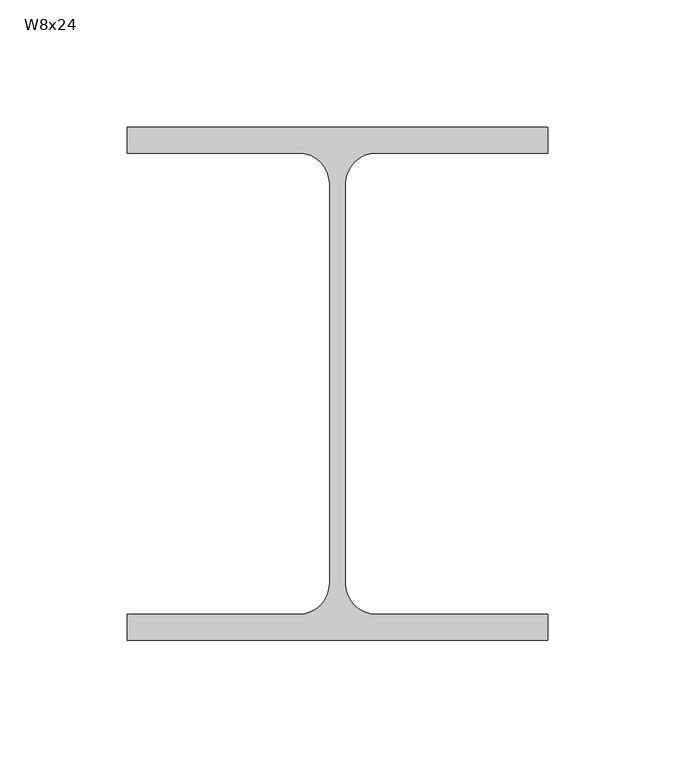
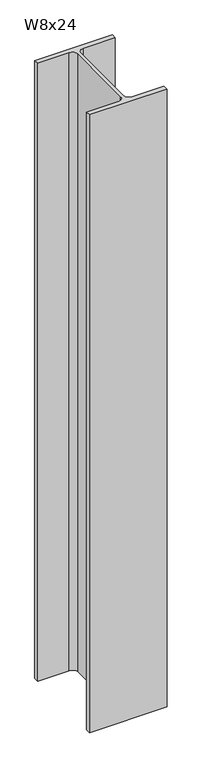
"""IFC4 building model written with IfcOpenShell, lengths in millimetres: column geometry, RME WF - Column : W8x24."""

from ifc_helpers import new_model, si_unit, point, frame, frame_2d, origin, place, context, project, spatial, polyline, circle_curve, trimmed, segment, composite_curve, outline, extrude, source, transform, mapped, element, save


def w8x24_9cd44bdc(model_context):
    return source(origin(), model_context, "Body", "SweptSolid", [
        extrude(outline(composite_curve([segment(polyline([(82.55, 100.711), (82.55, 90.551), (15.1765, 90.551)]), True, "CONTINUOUS"), segment(trimmed(circle_curve(frame_2d((15.1765, 78.486)), 12.065), [point((15.1765, 90.551))], [point((3.1115, 78.486))], True, "CARTESIAN"), True, "CONTINUOUS"), segment(polyline([(3.1115, 78.486), (3.1115, -78.486)]), True, "CONTINUOUS"), segment(trimmed(circle_curve(frame_2d((15.1765, -78.486)), 12.065), [point((3.1115, -78.486))], [point((15.1765, -90.551))], True, "CARTESIAN"), True, "CONTINUOUS"), segment(polyline([(15.1765, -90.551), (82.55, -90.551), (82.55, -100.711), (-82.55, -100.711), (-82.55, -90.551), (-15.1765, -90.551)]), True, "CONTINUOUS"), segment(trimmed(circle_curve(frame_2d((-15.1765, -78.486)), 12.065), [point((-15.1765, -90.551))], [point((-3.1115, -78.486))], True, "CARTESIAN"), True, "CONTINUOUS"), segment(polyline([(-3.1115, -78.486), (-3.1115, 78.486)]), True, "CONTINUOUS"), segment(trimmed(circle_curve(frame_2d((-15.1765, 78.486)), 12.065), [point((-3.1115, 78.486))], [point((-15.1765, 90.551))], True, "CARTESIAN"), True, "CONTINUOUS"), segment(polyline([(-15.1765, 90.551), (-82.55, 90.551), (-82.55, 100.711), (82.55, 100.711)]), True, "CONTINUOUS")], self_intersect=False)), frame((0.0, 0.0, 4699.0), z_axis=(0.0, 0.0, 1.0), x_axis=(1.0, 0.0, 0.0)), (0.0, 0.0, 1.0), 1390.65),
    ])


if __name__ == "__main__":
    model = new_model("IFC4")
    model_context = context("Model", 3, world=origin())
    ifc_project = project(units=[si_unit("LENGTHUNIT", "METRE", prefix="MILLI")], contexts=[model_context])
    site = spatial("IfcSite", under=ifc_project)
    building = spatial("IfcBuilding", under=site)
    placement = place(None, origin())
    w8x24_shape = w8x24_9cd44bdc(model_context)
    element("IfcColumn", 1, ObjectType="RME WF - Column : W8x24", at=placement, inside=building, context=model_context, shape_type="MappedRepresentation", body=[
        mapped(w8x24_shape, transform((0.0, 0.0, 0.0), x_axis=(1.0, 0.0, 0.0), y_axis=(0.0, 1.0, 0.0), z_axis=(0.0, 0.0, 1.0))),
    ])
    save(model, "model.ifc")

# Revit data of these elements
# Type "RME WF - Column : W8x24"
#   Type Mark = "C1"
#   REINF TYPE [instance default] = ""
#   Nominal Size = "W16"
#   COL REMARKS [instance default] = ""
#   BP [instance default] = ""
#   Assembly Code = "B10"
#   W = 24
#   bf = 0' - 6 1/2"
#   d = 0' - 7.93"
#   k = 0' - 0 7/8"
#   kr = 0' - 0.475"
#   tf = 0' - 0.4"
#   tw = 0' - 0.245"
#   A = 0.0491667 SF
#   Structural Material [instance default] = Metal - Steel - ASTM A992
# Element 1 (IfcColumn, "RME WF - Column : W8x24")
#   Materials on its faces: "Metal - Steel - ASTM A992"
# Materials
#   "Metal - Steel - ASTM A992": class "Metal", colour RGB 255 128 0, transparency 0
